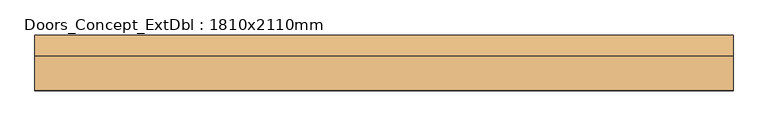
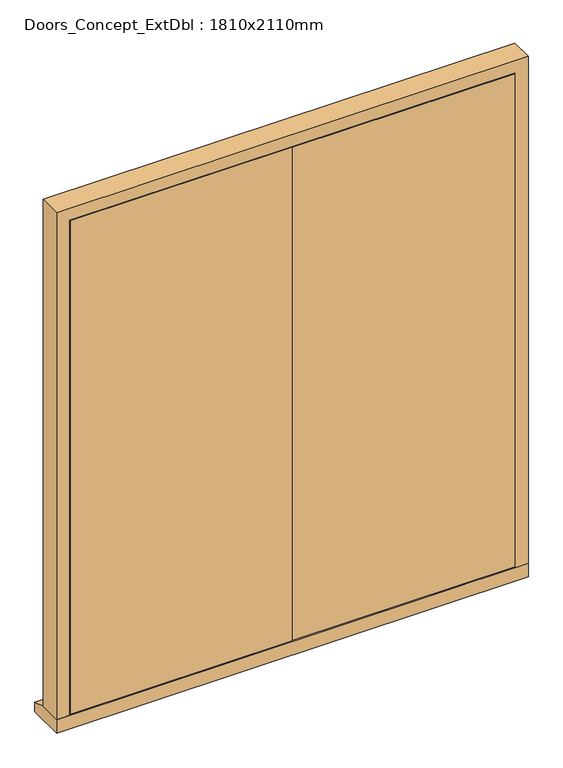
"""IFC4 building model written with IfcOpenShell, lengths in millimetres: door geometry, Doors_Concept_ExtDbl : 1810x2110mm."""

from ifc_helpers import new_model, si_unit, frame, origin, place, context, project, spatial, polyline, outline, extrude, faceted_brep, source, transform, mapped, element, save


def doors_concept_extdbl_1810x2110mm_b9f5cbc2(model_context):
    return source(origin(), model_context, "Body", "SolidModel", [
        faceted_brep([(834.5, 137.25, 54.5), (905.0, 137.25, 54.5), (905.0, 48.25, 54.5), (856.5, 48.25, 54.5), (856.5, 95.25, 54.5), (834.5, 95.25, 54.5), (834.5, 137.25, 2039.5), (-834.5, 137.25, 2039.5), (-834.5, 137.25, 54.5), (-905.0, 137.25, 54.5), (-905.0, 137.25, 2110.0), (905.0, 137.25, 2110.0), (905.0, 48.25, 2110.0), (-905.0, 48.25, 2110.0), (-905.0, 48.25, 54.5), (-856.5, 48.25, 54.5), (-856.5, 48.25, 2061.5), (856.5, 48.25, 2061.5), (856.5, 95.25, 2061.5), (-856.5, 95.25, 2061.5), (-856.5, 95.25, 54.5), (-834.5, 95.25, 54.5), (-834.5, 95.25, 2039.5), (834.5, 95.25, 2039.5)], [[[0, 1, 2, 3, 4, 5]], [[1, 0, 6, 7, 8, 9, 10, 11]], [[2, 1, 11, 12]], [[3, 2, 12, 13, 14, 15, 16, 17]], [[4, 3, 17, 18]], [[5, 4, 18, 19, 20, 21, 22, 23]], [[0, 5, 23, 6]], [[7, 22, 21, 8]], [[8, 21, 20, 15, 14, 9]], [[13, 10, 9, 14]], [[19, 16, 15, 20]], [[12, 11, 10, 13]], [[18, 17, 16, 19]], [[6, 23, 22, 7]]]),
        extrude(outline(polyline([(48.25, 0.0), (48.25, 54.5), (137.25, 54.5), (192.25, 38.5947221), (192.25, 0.0), (48.25, 0.0)])), frame((-905.0, 0.0, 0.0), z_axis=(1.0, 0.0, 0.0), x_axis=(0.0, 1.0, 0.0)), (0.0, 0.0, 1.0), 1810.0),
        extrude(outline(polyline([(853.5, 48.25), (1.5, 48.25), (1.5, 92.25), (853.5, 92.25), (853.5, 48.25)])), frame((0.0, 0.0, 58.5), z_axis=(0.0, 0.0, 1.0), x_axis=(1.0, 0.0, 0.0)), (0.0, 0.0, 1.0), 2000.0),
        extrude(outline(polyline([(-1.5, 48.25), (-853.5, 48.25), (-853.5, 92.25), (-1.5, 92.25), (-1.5, 48.25)])), frame((0.0, 0.0, 58.5), z_axis=(0.0, 0.0, 1.0), x_axis=(1.0, 0.0, 0.0)), (0.0, 0.0, 1.0), 2000.0),
    ])


if __name__ == "__main__":
    model = new_model("IFC4")
    model_context = context("Model", 3, world=origin())
    ifc_project = project(units=[si_unit("LENGTHUNIT", "METRE", prefix="MILLI")], contexts=[model_context])
    site = spatial("IfcSite", under=ifc_project)
    building = spatial("IfcBuilding", under=site)
    placement = place(None, origin())
    doors_concept_extdbl_1810x2110mm_shape = doors_concept_extdbl_1810x2110mm_b9f5cbc2(model_context)
    element("IfcDoor", 1, ObjectType="Doors_Concept_ExtDbl : 1810x2110mm", at=placement, inside=building, context=model_context, shape_type="MappedRepresentation", body=[
        mapped(doors_concept_extdbl_1810x2110mm_shape, transform((0.0, 0.0, 0.0), x_axis=(1.0, 0.0, 0.0), y_axis=(0.0, 1.0, 0.0), z_axis=(0.0, 0.0, 1.0))),
    ])
    save(model, "model.ifc")

# Revit data of these elements
# Type "Doors_Concept_ExtDbl : 1810x2110mm"
#   Type Mark = "47"
#   Type Comments = "External Double"
#   Operation = "DoubleDoorSingleSwing"
#   Construction Type Id = "GSP4R"
#   Keynote = "L10"
#   Analytic Construction = "1/8 in Pilkington single glazing"
#   Visual Light Transmittance = 0.9
#   Thickness = 44 mm
#   Solar Heat Gain Coefficient = 0.78
#   Rough Width = 1810 mm
#   Rough Height = 2110 mm
#   Heat Transfer Coefficient (U) = 3.6886 W/(m²·K)
#   FrameWidth = 42 mm
#   FrameOffset - External = 25 mm
#   Height = 2110 mm
#   Width = 1810 mm
#   Function = 1
#   Material Door = Concept
#   Material Frame = Concept
#   Wall Closure = (empty or 0)
# Element 1 (IfcDoor, "Doors_Concept_ExtDbl : 1810x2110mm")
#   Materials on its faces: "Concept"
# Materials
#   "Concept": class "Miscellaneous", colour RGB 128 128 255, transparency 0.5
